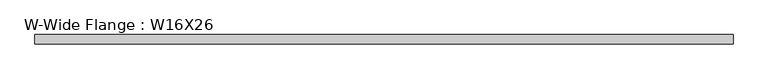
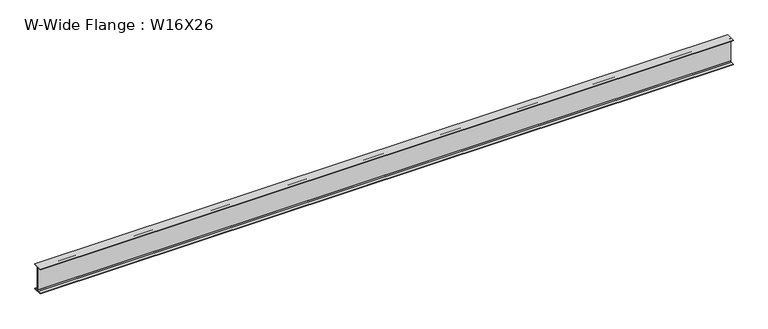
"""IFC4 building model written with IfcOpenShell, lengths in millimetres: beam geometry, W-Wide Flange : W16X26."""

from ifc_helpers import new_model, si_unit, point, frame, frame_2d, origin, place, context, project, spatial, polyline, circle_curve, trimmed, segment, composite_curve, outline, extrude, source, transform, mapped, element, save


def w_wide_flange_w16x26_a3dbe27b(model_context):
    return source(origin(), model_context, "Body", "SweptSolid", [
        extrude(outline(composite_curve([segment(polyline([(69.85, -190.627), (69.85, -199.39), (-69.85, -199.39), (-69.85, -190.627), (-21.3995, -190.627)]), True, "CONTINUOUS"), segment(trimmed(circle_curve(frame_2d((-21.3995, -172.4025)), 18.2245), [point((-21.3995, -190.627))], [point((-3.175, -172.4025))], True, "CARTESIAN"), True, "CONTINUOUS"), segment(polyline([(-3.175, -172.4025), (-3.175, 172.4025)]), True, "CONTINUOUS"), segment(trimmed(circle_curve(frame_2d((-21.3995, 172.4025)), 18.2245), [point((-3.175, 172.4025))], [point((-21.3995, 190.627))], True, "CARTESIAN"), True, "CONTINUOUS"), segment(polyline([(-21.3995, 190.627), (-69.85, 190.627), (-69.85, 199.39), (69.85, 199.39), (69.85, 190.627), (21.3995, 190.627)]), True, "CONTINUOUS"), segment(trimmed(circle_curve(frame_2d((21.3995, 172.4025)), 18.2245), [point((21.3995, 190.627))], [point((3.175, 172.4025))], True, "CARTESIAN"), True, "CONTINUOUS"), segment(polyline([(3.175, 172.4025), (3.175, -172.4025)]), True, "CONTINUOUS"), segment(trimmed(circle_curve(frame_2d((21.3995, -172.4025)), 18.2245), [point((3.175, -172.4025))], [point((21.3995, -190.627))], True, "CARTESIAN"), True, "CONTINUOUS"), segment(polyline([(21.3995, -190.627), (69.85, -190.627)]), True, "CONTINUOUS")], self_intersect=False)), frame((-5304.0661233, 0.0, 0.0), z_axis=(1.0, 0.0, 0.0), x_axis=(0.0, 1.0, 0.0)), (0.0, 0.0, 1.0), 10591.3863205),
    ])


if __name__ == "__main__":
    model = new_model("IFC4")
    model_context = context("Model", 3, world=origin())
    ifc_project = project(units=[si_unit("LENGTHUNIT", "METRE", prefix="MILLI")], contexts=[model_context])
    site = spatial("IfcSite", under=ifc_project)
    building = spatial("IfcBuilding", under=site)
    placement = place(None, origin())
    w_wide_flange_w16x26_shape = w_wide_flange_w16x26_a3dbe27b(model_context)
    element("IfcBeam", 1, ObjectType="W-Wide Flange : W16X26", at=placement, inside=building, context=model_context, shape_type="MappedRepresentation", body=[
        mapped(w_wide_flange_w16x26_shape, transform((0.0, 0.0, 0.0), x_axis=(1.0, 0.0, 0.0), y_axis=(0.0, 1.0, 0.0), z_axis=(0.0, 0.0, 1.0))),
    ])
    save(model, "model.ifc")

# Revit data of these elements
# Type "W-Wide Flange : W16X26"
#   Assembly Code = "B10"
#   W = 26
#   Length [instance default] = 5' - 0"
#   bf = 0' - 5 1/2"
#   d = 1' - 3.7"
#   k = 0' - 1 1/16"
#   k2 = 0' - 0.7175"
#   tf = 0' - 0.345"
#   tw = 0' - 0 1/4"
#   A = 0.0533333 SF
#   Structural Material [instance default] = Steel ASTM A992
# Element 1 (IfcBeam, "W-Wide Flange : W16X26")
#   Structural Material = Steel ASTM A36
#   Materials on its faces: "Steel ASTM A36"
# Materials
#   "Steel ASTM A992": class "Metal", colour RGB 199 199 199, transparency 0, Description = "Structural steel 50ksi", Cost = 0
#   "Steel ASTM A36": class "Metal", colour RGB 199 199 199, transparency 0, Description = "Structural steel, ASTM A36 Grade B, mill finish", Cost = 0
